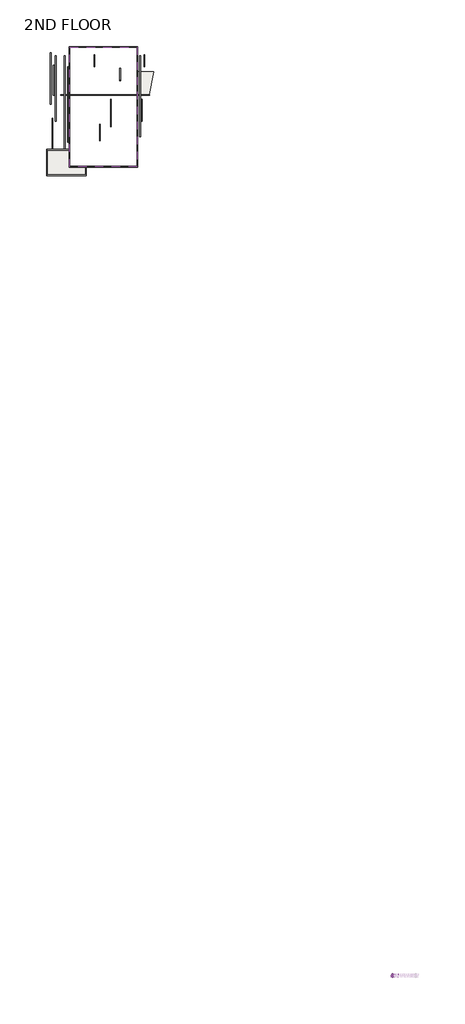
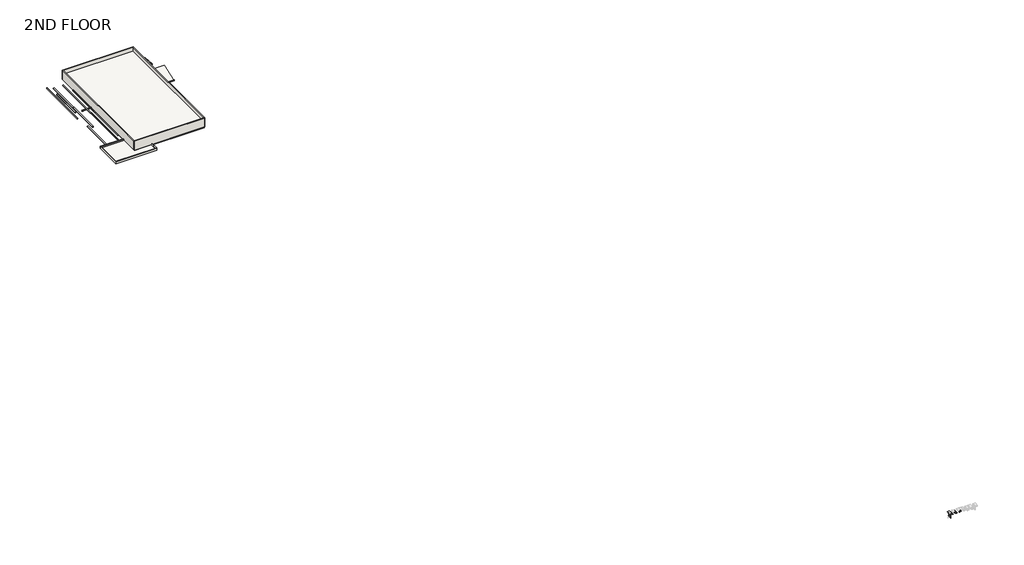
# One storey, part 1 of 2: 20 proxies, 18 beams, 8 walls, 3 slabs.
"""IFC4 building model written with IfcOpenShell, lengths in millimetres."""

import ifcopenshell
import ifcopenshell.guid

model = None  # the IFC model being written
_history = None  # IfcOwnerHistory: only IFC2X3 demands one
_inside = {}  # id of a spatial element -> (the spatial element, [elements in it])
_under = {}  # id of a project, library or spatial element -> (it, [spatial elements below it])
_declared = {}  # id of a project -> (the project, [libraries it declares])
_typed = {}  # id of a type object -> (the type object, [elements of that type])
_made_of = {}  # id of a material, layer set ... -> (it, [elements and type objects made of it])


def new_model(schema):
    """Start an empty IFC model of exactly this schema.

    Asked for "IFC4X3", IfcOpenShell would pick the latest addendum, in which some entities
    have other attributes; the version numbers below select the first issue.
    IFC2X3 requires an IfcOwnerHistory on every rooted entity: one is made here for all.
    """
    global model, _history
    if schema == "IFC4X3":
        model = ifcopenshell.file(schema_version=(4, 3, 0, 0))
    else:
        model = ifcopenshell.file(schema=schema)
    _inside.clear()
    _under.clear()
    _declared.clear()
    _typed.clear()
    _made_of.clear()
    _history = None
    if model.schema == "IFC2X3":
        org = make("IfcOrganization", Name="unknown")
        user = make(
            "IfcPersonAndOrganization",
            ThePerson=make("IfcPerson", FamilyName="unknown"),
            TheOrganization=org,
        )
        app = make(
            "IfcApplication",
            ApplicationDeveloper=org,
            Version="unknown",
            ApplicationFullName="unknown",
            ApplicationIdentifier="unknown",
        )
        _history = make(
            "IfcOwnerHistory",
            OwningUser=user,
            OwningApplication=app,
            ChangeAction="ADDED",
            CreationDate=0,
        )
    return model


def make(cls, **values):
    """One entity of the class cls with the attributes given. An attribute that is None is left unset."""
    return model.create_entity(
        cls, **{name: value for name, value in values.items() if value is not None}
    )


def rooted(cls, **values):
    """An entity with a GlobalId (a new one), such as an element, a storey or a relation."""
    return make(cls, GlobalId=ifcopenshell.guid.new(), OwnerHistory=_history, **values)


def si_unit(unit_type, name, prefix=None):
    """IfcSIUnit, for example si_unit("LENGTHUNIT", "METRE", prefix="MILLI")."""
    return make("IfcSIUnit", UnitType=unit_type, Prefix=prefix, Name=name)


def assignment(units):
    """IfcUnitAssignment: the units of a project."""
    return None if units is None else make("IfcUnitAssignment", Units=units)


def point(xyz):
    """IfcCartesianPoint."""
    return None if xyz is None else make("IfcCartesianPoint", Coordinates=xyz)


def direction(xyz):
    """IfcDirection."""
    return None if xyz is None else make("IfcDirection", DirectionRatios=xyz)


def frame(location, z_axis=None, x_axis=None):
    """IfcAxis2Placement3D, a coordinate frame: its origin and axes. An axis left out is left unset."""
    return make(
        "IfcAxis2Placement3D",
        Location=point(location),
        Axis=direction(z_axis),
        RefDirection=direction(x_axis),
    )


def frame_2d(location, x_axis=None):
    """IfcAxis2Placement2D, a coordinate frame in the plane: its origin and x axis."""
    return make(
        "IfcAxis2Placement2D", Location=point(location), RefDirection=direction(x_axis)
    )


def origin():
    """The frame at (0, 0, 0) with its axes left unset."""
    return frame((0.0, 0.0, 0.0))


def place(relative_to, where):
    """IfcLocalPlacement: puts the frame where relative to a parent placement (None: the world)."""
    return make(
        "IfcLocalPlacement", PlacementRelTo=relative_to, RelativePlacement=where
    )


def context(
    kind, dimensions, precision=None, world=None, true_north=None, identifier=None
):
    """IfcGeometricRepresentationContext, for example the 3D "Model" context."""
    return make(
        "IfcGeometricRepresentationContext",
        ContextIdentifier=identifier,
        ContextType=kind,
        CoordinateSpaceDimension=dimensions,
        Precision=precision,
        WorldCoordinateSystem=world,
        TrueNorth=true_north,
    )


def project(units=None, contexts=None):
    """IfcProject with its units and contexts."""
    return rooted(
        "IfcProject",
        Name="project",
        RepresentationContexts=contexts,
        UnitsInContext=assignment(units),
    )


def spatial(cls, under=None, at=None, **own):
    """A site, building, storey or space (cls), placed at a placement, below another one or the project."""
    s = rooted(cls, ObjectPlacement=at, **own)
    if under is not None:
        _under.setdefault(under.id(), (under, []))[1].append(s)
    return s


def polyline(points):
    """IfcPolyline through the points."""
    return make("IfcPolyline", Points=[point(p) for p in points])


def circle_curve(where, radius):
    """IfcCircle in the frame where."""
    return make("IfcCircle", Position=where, Radius=radius)


def trimmed(basis, trim1, trim2, sense, master):
    """IfcTrimmedCurve: the piece of a basis curve between two trims."""
    return make(
        "IfcTrimmedCurve",
        BasisCurve=basis,
        Trim1=trim1,
        Trim2=trim2,
        SenseAgreement=sense,
        MasterRepresentation=master,
    )


def segment(curve, same_sense, transition):
    """IfcCompositeCurveSegment."""
    return make(
        "IfcCompositeCurveSegment",
        Transition=transition,
        SameSense=same_sense,
        ParentCurve=curve,
    )


def composite_curve(segments, self_intersect=None):
    """IfcCompositeCurve: segments joined end to end."""
    return make("IfcCompositeCurve", Segments=segments, SelfIntersect=self_intersect)


def outline(outer, holes=None, kind="AREA"):
    """IfcArbitraryClosedProfileDef: a profile drawn as a closed curve; with holes, ...WithVoids."""
    if holes is None:
        return make("IfcArbitraryClosedProfileDef", ProfileType=kind, OuterCurve=outer)
    return make(
        "IfcArbitraryProfileDefWithVoids",
        ProfileType=kind,
        OuterCurve=outer,
        InnerCurves=holes,
    )


def extrude(swept, where, along, depth):
    """IfcExtrudedAreaSolid: the profile swept, set in the frame where, extruded along a direction by depth."""
    return make(
        "IfcExtrudedAreaSolid",
        SweptArea=swept,
        Position=where,
        ExtrudedDirection=direction(along),
        Depth=depth,
    )


def faces_of(points, faces, orient=None, outer=None):
    """IfcFace entities. A face is a list of loops; a loop is a list of indices into points, from 0.

    orient and outer hold one flag for each loop. By default every Orientation is true, the
    first loop of a face is its IfcFaceOuterBound and the others are IfcFaceBound.
    """
    made = []
    for i, loops in enumerate(faces):
        bounds = []
        for j, loop in enumerate(loops):
            is_outer = j == 0 if outer is None else outer[i][j]
            bounds.append(
                make(
                    "IfcFaceOuterBound" if is_outer else "IfcFaceBound",
                    Bound=make("IfcPolyLoop", Polygon=[points[k] for k in loop]),
                    Orientation=True if orient is None else orient[i][j],
                )
            )
        made.append(make("IfcFace", Bounds=bounds))
    return made


def faceted_brep(points, faces, orient=None, outer=None, voids=None):
    """IfcFacetedBrep: a solid bounded by flat faces; with voids (closed shells), ...WithVoids."""
    shared = [point(p) for p in points]
    hull = make("IfcClosedShell", CfsFaces=faces_of(shared, faces, orient, outer))
    if voids is None:
        return make("IfcFacetedBrep", Outer=hull)
    return make(
        "IfcFacetedBrepWithVoids",
        Outer=hull,
        Voids=[
            make(cls, CfsFaces=faces_of(shared, fs, o, b)) for cls, fs, o, b in voids
        ],
    )


def shape(context_of_items, identifier, shape_type, items):
    """IfcShapeRepresentation: the items that make up one representation, for example the "Body"."""
    return make(
        "IfcShapeRepresentation",
        ContextOfItems=context_of_items,
        RepresentationIdentifier=identifier,
        RepresentationType=shape_type,
        Items=items,
    )


def source(mapping_origin, context_of_items, identifier, shape_type, items):
    """IfcRepresentationMap: a shape defined once, which mapped items show again and again."""
    return make(
        "IfcRepresentationMap",
        MappingOrigin=mapping_origin,
        MappedRepresentation=shape(context_of_items, identifier, shape_type, items),
    )


def transform(
    local_origin,
    x_axis=None,
    y_axis=None,
    z_axis=None,
    scale=None,
    scale2=None,
    scale3=None,
    uniform=True,
):
    """IfcCartesianTransformationOperator3D, or its non-uniform kind. x_axis, y_axis, z_axis: its Axis1, 2, 3."""
    if uniform:
        return make(
            "IfcCartesianTransformationOperator3D",
            Axis1=direction(x_axis),
            Axis2=direction(y_axis),
            LocalOrigin=point(local_origin),
            Scale=scale,
            Axis3=direction(z_axis),
        )
    return make(
        "IfcCartesianTransformationOperator3DnonUniform",
        Axis1=direction(x_axis),
        Axis2=direction(y_axis),
        LocalOrigin=point(local_origin),
        Scale=scale,
        Axis3=direction(z_axis),
        Scale2=scale2,
        Scale3=scale3,
    )


def mapped(mapping_source, mapping_target):
    """IfcMappedItem: shows the shape of a source again, moved by a transform."""
    return make(
        "IfcMappedItem", MappingSource=mapping_source, MappingTarget=mapping_target
    )


def made_of(thing, what):
    """Note that an element or type object is made of a material, layer set ...; save() writes the relation."""
    if what is not None:
        _made_of.setdefault(what.id(), (what, []))[1].append(thing)
    return thing


def element(
    cls,
    number,
    at=None,
    inside=None,
    cuts=None,
    type_object=None,
    material=None,
    context=None,
    identifier="Body",
    shape_type=None,
    held_by="IfcProductDefinitionShape",
    body=None,
    shapes=None,
    **own,
):
    """One element of the class cls, such as IfcWall. Its Tag is "e" and its number.

    at: its placement. inside: the storey or other place that contains it. cuts: it is an
    opening in that element (IfcRelVoidsElement). A single representation is given by context,
    identifier, shape_type and body (its items); several are given by shapes. held_by: the class
    of the entity that holds the representations. save() writes the other relations.
    """
    e = rooted(cls, Tag="e%d" % number, ObjectPlacement=at, **own)
    if body is not None:
        shapes = [shape(context, identifier, shape_type, body)]
    if shapes is not None:
        e.Representation = make(held_by, Representations=shapes)
    if inside is not None:
        _inside.setdefault(inside.id(), (inside, []))[1].append(e)
    if cuts is not None:
        rooted(
            "IfcRelVoidsElement", RelatingBuildingElement=cuts, RelatedOpeningElement=e
        )
    if type_object is not None:
        _typed.setdefault(type_object.id(), (type_object, []))[1].append(e)
    return made_of(e, material)


def aggregate(whole, parts):
    """IfcRelAggregates: a whole, such as a stair, and the parts it consists of."""
    return rooted("IfcRelAggregates", RelatingObject=whole, RelatedObjects=parts)


def save(model, path):
    """Write the relations noted so far, then the file.

    IfcRelAggregates (storeys below a building ...), IfcRelContainedInSpatialStructure (elements
    in a storey), IfcRelDefinesByType, IfcRelAssociatesMaterial and IfcRelDeclares: one each for
    every whole, place, type object, material and project.
    """
    for whole, parts in _under.values():
        aggregate(whole, parts)
    for where, things in _inside.values():
        rooted(
            "IfcRelContainedInSpatialStructure",
            RelatedElements=things,
            RelatingStructure=where,
        )
    for kind, things in _typed.values():
        rooted("IfcRelDefinesByType", RelatedObjects=things, RelatingType=kind)
    for what, things in _made_of.values():
        rooted("IfcRelAssociatesMaterial", RelatedObjects=things, RelatingMaterial=what)
    for by, libraries in _declared.values():
        rooted("IfcRelDeclares", RelatingContext=by, RelatedDefinitions=libraries)
    model.write(path)


def dimension_lumber_10x10_beam_780dcf97(model_context):
    return source(origin(), model_context, "Body", "SweptSolid", [
        extrude(outline(polyline([(3429.0, 117.475), (3429.0, -117.475), (-3429.0, -117.475), (-3429.0, 117.475), (3429.0, 117.475)])), frame((0.0, 0.0, -117.475), z_axis=(0.0, 0.0, 1.0), x_axis=(1.0, 0.0, 0.0)), (0.0, 0.0, 1.0), 234.95),
    ])


def dimension_lumber_10x10_beam_a659b46f(model_context):
    return source(origin(), model_context, "Body", "SweptSolid", [
        extrude(outline(polyline([(11658.6, 117.475), (11658.6, -117.475), (-11658.6, -117.475), (-11658.6, 117.475), (11658.6, 117.475)])), frame((0.0, 0.0, -117.475), z_axis=(0.0, 0.0, 1.0), x_axis=(1.0, 0.0, 0.0)), (0.0, 0.0, 1.0), 234.95),
    ])


def dimension_lumber_10x10_beam_82f4ea42(model_context):
    return source(origin(), model_context, "Body", "SweptSolid", [
        extrude(outline(polyline([(4648.2, 117.475), (4648.2, -117.475), (-4648.2, -117.475), (-4648.2, 117.475), (4648.2, 117.475)])), frame((0.0, 0.0, -117.475), z_axis=(0.0, 0.0, 1.0), x_axis=(1.0, 0.0, 0.0)), (0.0, 0.0, 1.0), 234.95),
    ])


def dimension_lumber_10x10_beam_babce44f(model_context):
    return source(origin(), model_context, "Body", "SweptSolid", [
        extrude(outline(polyline([(7924.8, 117.475), (7924.8, -117.475), (-7924.8, -117.475), (-7924.8, 117.475), (7924.8, 117.475)])), frame((0.0, 0.0, -117.475), z_axis=(0.0, 0.0, 1.0), x_axis=(1.0, 0.0, 0.0)), (0.0, 0.0, 1.0), 234.95),
    ])


def dimension_lumber_10x10_beam_47096931(model_context):
    return source(origin(), model_context, "Body", "SweptSolid", [
        extrude(outline(polyline([(10420.9864513, 117.475), (10420.9864513, -117.475), (-10420.9864513, -117.475), (-10420.9864513, 117.475), (10420.9864513, 117.475)])), frame((0.0, 0.0, -117.475), z_axis=(0.0, 0.0, 1.0), x_axis=(1.0, 0.0, 0.0)), (0.0, 0.0, 1.0), 234.95),
    ])


def dimension_lumber_10x10_beam_db3298f4(model_context):
    return source(origin(), model_context, "Body", "SweptSolid", [
        extrude(outline(polyline([(12496.8, 117.475), (12496.8, -117.475), (-12496.8, -117.475), (-12496.8, 117.475), (12496.8, 117.475)])), frame((0.0, 0.0, -117.475), z_axis=(0.0, 0.0, 1.0), x_axis=(1.0, 0.0, 0.0)), (0.0, 0.0, 1.0), 234.95),
    ])


def dimension_lumber_10x10_beam_470fd3cf(model_context):
    return source(origin(), model_context, "Body", "SweptSolid", [
        extrude(outline(polyline([(1876.3363558, 117.475), (1876.3363558, -117.475), (-1876.3363558, -117.475), (-1876.3363558, 117.475), (1876.3363558, 117.475)])), frame((0.0, 0.0, -117.475), z_axis=(0.0, 0.0, 1.0), x_axis=(1.0, 0.0, 0.0)), (0.0, 0.0, 1.0), 234.95),
    ])


def dimension_lumber_10x10_beam_1dfca716(model_context):
    return source(origin(), model_context, "Body", "SweptSolid", [
        extrude(outline(polyline([(10094.9494295, 117.475), (10094.9494295, -117.475), (-10094.9494295, -117.475), (-10094.9494295, 117.475), (10094.9494295, 117.475)])), frame((0.0, 0.0, -117.475), z_axis=(0.0, 0.0, 1.0), x_axis=(1.0, 0.0, 0.0)), (0.0, 0.0, 1.0), 234.95),
    ])


def dimension_lumber_10x10_beam_bd205abd(model_context):
    return source(origin(), model_context, "Body", "SweptSolid", [
        extrude(outline(polyline([(14564.075555, 117.475), (14564.075555, -117.475), (-14467.238055, -117.475), (-14467.238055, 117.475), (14564.075555, 117.475)])), frame((0.0, 0.0, -117.475), z_axis=(0.0, 0.0, 1.0), x_axis=(1.0, 0.0, 0.0)), (0.0, 0.0, 1.0), 234.95),
    ])


def dimension_lumber_10x10_beam_e017d86a(model_context):
    return source(origin(), model_context, "Body", "SweptSolid", [
        extrude(outline(polyline([(4267.2, 117.475), (4267.2, -117.475), (-4267.2, -117.475), (-4267.2, 117.475), (4267.2, 117.475)])), frame((0.0, 0.0, -117.475), z_axis=(0.0, 0.0, 1.0), x_axis=(1.0, 0.0, 0.0)), (0.0, 0.0, 1.0), 234.95),
    ])


def dimension_lumber_10x10_beam_f930df24(model_context):
    return source(origin(), model_context, "Body", "SweptSolid", [
        extrude(outline(polyline([(2514.6, 117.475), (2514.6, -117.475), (-2514.6, -117.475), (-2514.6, 117.475), (2514.6, 117.475)])), frame((0.0, 0.0, -117.475), z_axis=(0.0, 0.0, 1.0), x_axis=(1.0, 0.0, 0.0)), (0.0, 0.0, 1.0), 234.95),
    ])


def w_wide_flange_w12x26_f67572b3(model_context):
    return source(origin(), model_context, "Body", "SweptSolid", [
        extrude(outline(composite_curve([segment(polyline([(82.4011719, -145.5539063), (82.4011719, -155.178125), (-82.4011719, -155.178125), (-82.4011719, -145.5539063), (-20.2902344, -145.5539063)]), True, "CONTINUOUS"), segment(trimmed(circle_curve(frame_2d((-20.2902344, -128.190625)), 17.3632812), [point((-20.2902344, -145.5539063))], [point((-2.9269531, -128.190625))], True, "CARTESIAN"), True, "CONTINUOUS"), segment(polyline([(-2.9269531, -128.190625), (-2.9269531, 128.190625)]), True, "CONTINUOUS"), segment(trimmed(circle_curve(frame_2d((-20.2902344, 128.190625)), 17.3632812), [point((-2.9269531, 128.190625))], [point((-20.2902344, 145.5539062))], True, "CARTESIAN"), True, "CONTINUOUS"), segment(polyline([(-20.2902344, 145.5539062), (-82.4011719, 145.5539062), (-82.4011719, 155.178125), (82.4011719, 155.178125), (82.4011719, 145.5539062), (20.2902344, 145.5539062)]), True, "CONTINUOUS"), segment(trimmed(circle_curve(frame_2d((20.2902344, 128.190625)), 17.3632812), [point((20.2902344, 145.5539062))], [point((2.9269531, 128.190625))], True, "CARTESIAN"), True, "CONTINUOUS"), segment(polyline([(2.9269531, 128.190625), (2.9269531, -128.190625)]), True, "CONTINUOUS"), segment(trimmed(circle_curve(frame_2d((20.2902344, -128.190625)), 17.3632812), [point((2.9269531, -128.190625))], [point((20.2902344, -145.5539063))], True, "CARTESIAN"), True, "CONTINUOUS"), segment(polyline([(20.2902344, -145.5539063), (82.4011719, -145.5539063)]), True, "CONTINUOUS")], self_intersect=False)), frame((-18489.1180586, 0.0, 0.0), z_axis=(1.0, 0.0, 0.0), x_axis=(0.0, 1.0, 0.0)), (0.0, 0.0, 1.0), 36978.2361173),
    ])


def w_wide_flange_w12x26_0a813f0e(model_context):
    return source(origin(), model_context, "Body", "SweptSolid", [
        extrude(outline(composite_curve([segment(polyline([(82.4011719, -145.5539063), (82.4011719, -155.178125), (-82.4011719, -155.178125), (-82.4011719, -145.5539063), (-20.2902344, -145.5539063)]), True, "CONTINUOUS"), segment(trimmed(circle_curve(frame_2d((-20.2902344, -128.190625)), 17.3632812), [point((-20.2902344, -145.5539063))], [point((-2.9269531, -128.190625))], True, "CARTESIAN"), True, "CONTINUOUS"), segment(polyline([(-2.9269531, -128.190625), (-2.9269531, 128.190625)]), True, "CONTINUOUS"), segment(trimmed(circle_curve(frame_2d((-20.2902344, 128.190625)), 17.3632812), [point((-2.9269531, 128.190625))], [point((-20.2902344, 145.5539062))], True, "CARTESIAN"), True, "CONTINUOUS"), segment(polyline([(-20.2902344, 145.5539062), (-82.4011719, 145.5539062), (-82.4011719, 155.178125), (82.4011719, 155.178125), (82.4011719, 145.5539062), (20.2902344, 145.5539062)]), True, "CONTINUOUS"), segment(trimmed(circle_curve(frame_2d((20.2902344, 128.190625)), 17.3632812), [point((20.2902344, 145.5539062))], [point((2.9269531, 128.190625))], True, "CARTESIAN"), True, "CONTINUOUS"), segment(polyline([(2.9269531, 128.190625), (2.9269531, -128.190625)]), True, "CONTINUOUS"), segment(trimmed(circle_curve(frame_2d((20.2902344, -128.190625)), 17.3632812), [point((2.9269531, -128.190625))], [point((20.2902344, -145.5539063))], True, "CARTESIAN"), True, "CONTINUOUS"), segment(polyline([(20.2902344, -145.5539063), (82.4011719, -145.5539063)]), True, "CONTINUOUS")], self_intersect=False)), frame((-25624.0113662, 0.0, 0.0), z_axis=(1.0, 0.0, 0.0), x_axis=(0.0, 1.0, 0.0)), (0.0, 0.0, 1.0), 27573.8603238),
    ])


def w_wide_flange_w12x26_89544ef1(model_context):
    return source(origin(), model_context, "Body", "SweptSolid", [
        extrude(outline(composite_curve([segment(polyline([(82.4011719, -145.5539063), (82.4011719, -155.178125), (-82.4011719, -155.178125), (-82.4011719, -145.5539063), (-20.2902344, -145.5539063)]), True, "CONTINUOUS"), segment(trimmed(circle_curve(frame_2d((-20.2902344, -128.190625)), 17.3632812), [point((-20.2902344, -145.5539063))], [point((-2.9269531, -128.190625))], True, "CARTESIAN"), True, "CONTINUOUS"), segment(polyline([(-2.9269531, -128.190625), (-2.9269531, 128.190625)]), True, "CONTINUOUS"), segment(trimmed(circle_curve(frame_2d((-20.2902344, 128.190625)), 17.3632812), [point((-2.9269531, 128.190625))], [point((-20.2902344, 145.5539062))], True, "CARTESIAN"), True, "CONTINUOUS"), segment(polyline([(-20.2902344, 145.5539062), (-82.4011719, 145.5539062), (-82.4011719, 155.178125), (82.4011719, 155.178125), (82.4011719, 145.5539062), (20.2902344, 145.5539062)]), True, "CONTINUOUS"), segment(trimmed(circle_curve(frame_2d((20.2902344, 128.190625)), 17.3632812), [point((20.2902344, 145.5539062))], [point((2.9269531, 128.190625))], True, "CARTESIAN"), True, "CONTINUOUS"), segment(polyline([(2.9269531, 128.190625), (2.9269531, -128.190625)]), True, "CONTINUOUS"), segment(trimmed(circle_curve(frame_2d((20.2902344, -128.190625)), 17.3632812), [point((2.9269531, -128.190625))], [point((20.2902344, -145.5539063))], True, "CARTESIAN"), True, "CONTINUOUS"), segment(polyline([(20.2902344, -145.5539063), (82.4011719, -145.5539063)]), True, "CONTINUOUS")], self_intersect=False)), frame((-18440.6993086, 0.0, 0.0), z_axis=(1.0, 0.0, 0.0), x_axis=(0.0, 1.0, 0.0)), (0.0, 0.0, 1.0), 36978.2361173),
    ])


def generic_models_1_generic_models_1_05f3df34(model_context):
    return source(origin(), model_context, "Body", "SweptSolid", [
        extrude(outline(polyline([(49784.0, 0.0), (49695.1, 0.0), (49695.1, 1219.2), (49784.0, 1219.2), (49784.0, 0.0)])), frame((0.0, 0.0, 3048.0), z_axis=(0.0, 0.0, 1.0), x_axis=(1.0, 0.0, 0.0)), (0.0, 0.0, 1.0), 38.1),
    ])


def generic_models_157_generic_models_1_b3b9a6c0(model_context):
    return source(origin(), model_context, "Body", "SweptSolid", [
        extrude(outline(polyline([(47363.0625, 1219.2), (47363.0625, 0.0), (47347.1875, 0.0), (47347.1875, 1219.2), (47363.0625, 1219.2)])), frame((0.0, 0.0, 4267.2), z_axis=(0.0, 0.0, 1.0), x_axis=(1.0, 0.0, 0.0)), (0.0, 0.0, 1.0), 1123.95),
    ])


def generic_models_14_generic_models_1_e8c90d4c(model_context):
    return source(origin(), model_context, "Body", "SweptSolid", [
        extrude(outline(polyline([(2277.1204978, 49799.875), (2239.0204978, 49799.875), (2239.0204978, 49825.275), (2240.6079978, 49825.275), (2240.6079978, 49801.4625), (2277.1204978, 49801.4625), (2277.1204978, 49799.875)])), frame((0.0, 0.0, 0.0), z_axis=(0.0, 1.0, 0.0), x_axis=(0.0, 0.0, 1.0)), (0.0, 0.0, 1.0), 1219.2),
    ])


def generic_models_22_generic_models_1_e5767157(model_context):
    return source(origin(), model_context, "Body", "SweptSolid", [
        extrude(outline(polyline([(2409.6091, 49800.66875), (2409.6091, 49799.875), (2407.0592364, 49799.875), (2405.4618473, 49749.075), (2404.6631527, 49749.075), (2403.0657636, 49799.875), (2400.5159, 49799.875), (2400.5159, 49800.66875), (2409.6091, 49800.66875)])), frame((0.0, 565.15, 0.0), z_axis=(0.0, 1.0, 0.0), x_axis=(0.0, 0.0, 1.0)), (0.0, 0.0, 1.0), 12.7),
    ])


def generic_models_226_generic_models_1_7dc37832(model_context):
    return source(origin(), model_context, "Body", "SweptSolid", [
        extrude(outline(polyline([(5263.35625, 49733.4159), (5263.35625, 49742.5091), (5264.15, 49742.5091), (5264.15, 49739.9592364), (5314.95, 49738.3618473), (5314.95, 49737.5631527), (5264.15, 49735.9657636), (5264.15, 49733.4159), (5263.35625, 49733.4159)])), frame((0.0, 565.15, 0.0), z_axis=(0.0, 1.0, 0.0), x_axis=(0.0, 0.0, 1.0)), (0.0, 0.0, 1.0), 12.7),
    ])


def generic_models_202_generic_models_1_0ad20a8b(model_context):
    return source(origin(), model_context, "Body", "SweptSolid", [
        extrude(outline(polyline([(2253.330428, 49813.3451407), (2242.217928, 49813.3451407), (2242.217928, 49826.0451407), (2234.280428, 49828.9341545), (2234.280428, 50422.9451407), (2253.330428, 50422.9451407), (2253.330428, 49813.3451407)])), frame((0.0, 0.0, 0.0), z_axis=(0.0, 1.0, 0.0), x_axis=(0.0, 0.0, 1.0)), (0.0, 0.0, 1.0), 1219.2),
    ])


def generic_models_239_generic_models_46_95e6735a(model_context):
    return source(origin(), model_context, "Body", "SweptSolid", [
        extrude(outline(polyline([(50347.5625, 0.0), (49691.4320511, 0.0), (49691.4320511, 1219.2), (50347.5625, 1219.2), (50347.5625, 0.0)])), frame((0.0, 0.0, 5505.7509163), z_axis=(0.0, 0.0, 1.0), x_axis=(1.0, 0.0, 0.0)), (0.0, 0.0, 1.0), 1.5875),
    ])


def generic_models_233_generic_models_1_ae5bae41(model_context):
    return source(origin(), model_context, "Body", "SweptSolid", [
        extrude(outline(polyline([(48564.8, 0.0), (48475.9, 0.0), (48475.9, 1219.2), (48564.8, 1219.2), (48564.8, 0.0)])), frame((0.0, 0.0, 5467.35), z_axis=(0.0, 0.0, 1.0), x_axis=(1.0, 0.0, 0.0)), (0.0, 0.0, 1.0), 38.1),
    ])


def generic_models_237_generic_models_65_1df05f16(model_context):
    return source(origin(), model_context, "Body", "SweptSolid", [
        extrude(outline(polyline([(48469.55, 592.1375), (48469.55, 630.2375), (49128.3625, 630.2375), (49128.3625, 592.1375), (48469.55, 592.1375)])), frame((0.0, 0.0, 5507.83125), z_axis=(0.0, 0.0, 1.0), x_axis=(1.0, 0.0, 0.0)), (0.0, 0.0, 1.0), 139.7),
    ])


def generic_models_240_generic_models_1_611786cf(model_context):
    return source(origin(), model_context, "Body", "SweptSolid", [
        extrude(outline(polyline([(49128.3625, 1219.2), (49128.3625, 0.0), (48469.55, 0.0), (48469.55, 1219.2), (49128.3625, 1219.2)])), frame((0.0, 0.0, 5649.9125), z_axis=(0.0, 0.0, 1.0), x_axis=(1.0, 0.0, 0.0)), (0.0, 0.0, 1.0), 19.05),
    ])


model = new_model("IFC4")

# Units and contexts
model_context = context("Model", 3, world=origin())
ifc_project = project(units=[si_unit("LENGTHUNIT", "METRE", prefix="MILLI")], contexts=[model_context])

# Site, building, storey
site = spatial("IfcSite", under=ifc_project)
building = spatial("IfcBuilding", under=site)
storey = spatial("IfcBuildingStorey", under=building, Name="2ND FLOOR", Elevation=3657.6)

# Beams
placement = place(None, origin())
dimension_lumber_10x10_beam_shape = dimension_lumber_10x10_beam_780dcf97(model_context)
element("IfcBeam", 1, ObjectType="Dimension Lumber : 10x10 - BEAM", at=placement, inside=storey, context=model_context, shape_type="MappedRepresentation", body=[
    mapped(dimension_lumber_10x10_beam_shape, transform((-31351.8083583, 267736.5959777, 4098.925), x_axis=(0.0, 1.0, 0.0), y_axis=(-1.0, 0.0, 0.0), z_axis=(0.0, 0.0, 1.0))),
])
dimension_lumber_10x10_beam_2_shape = dimension_lumber_10x10_beam_a659b46f(model_context)
element("IfcBeam", 2, ObjectType="Dimension Lumber : 10x10 - BEAM", at=placement, inside=storey, context=model_context, shape_type="MappedRepresentation", body=[
    mapped(dimension_lumber_10x10_beam_2_shape, transform((-54174.023811, 269565.3959777, 4098.925), x_axis=(0.0, 1.0, 0.0), y_axis=(-1.0, 0.0, 0.0), z_axis=(0.0, 0.0, 1.0))),
])
dimension_lumber_10x10_beam_3_shape = dimension_lumber_10x10_beam_82f4ea42(model_context)
element("IfcBeam", 3, ObjectType="Dimension Lumber : 10x10 - BEAM", at=placement, inside=storey, context=model_context, shape_type="MappedRepresentation", body=[
    mapped(dimension_lumber_10x10_beam_3_shape, transform((-58593.623811, 277032.9959777, 4098.925), x_axis=(0.0, 1.0, 0.0), y_axis=(-1.0, 0.0, 0.0), z_axis=(0.0, 0.0, 1.0))),
])
element("IfcBeam", 4, ObjectType="Dimension Lumber : 10x10 - BEAM", at=placement, inside=storey, context=model_context, shape_type="MappedRepresentation", body=[
    mapped(dimension_lumber_10x10_beam_3_shape, transform((-58989.4061381, 260573.7959777, 4098.925), x_axis=(0.0, 1.0, 0.0), y_axis=(-1.0, 0.0, 0.0), z_axis=(0.0, 0.0, 1.0))),
])
dimension_lumber_10x10_beam_4_shape = dimension_lumber_10x10_beam_babce44f(model_context)
element("IfcBeam", 5, ObjectType="Dimension Lumber : 10x10 - BEAM", at=placement, inside=storey, context=model_context, shape_type="MappedRepresentation", body=[
    mapped(dimension_lumber_10x10_beam_4_shape, transform((-59508.023811, 277566.3959777, 4098.925), x_axis=(0.0, 1.0, 0.0), y_axis=(-1.0, 0.0, 0.0), z_axis=(0.0, 0.0, 1.0))),
])
dimension_lumber_10x10_beam_5_shape = dimension_lumber_10x10_beam_47096931(model_context)
element("IfcBeam", 6, ObjectType="Dimension Lumber : 10x10 - BEAM", at=placement, inside=storey, context=model_context, shape_type="MappedRepresentation", body=[
    mapped(dimension_lumber_10x10_beam_5_shape, transform((-43244.9562094, 250288.6950863, 3844.925), x_axis=(1.0, 0.0, 0.0), y_axis=(0.0, 1.0, 0.0), z_axis=(0.0, 0.0, 1.0))),
])
element("IfcBeam", 7, ObjectType="Dimension Lumber : 10x10 - BEAM", at=placement, inside=storey, context=model_context, shape_type="MappedRepresentation", body=[
    mapped(dimension_lumber_10x10_beam_5_shape, transform((-43244.9562094, 287271.6937036, 3844.925), x_axis=(1.0, 0.0, 0.0), y_axis=(0.0, 1.0, 0.0), z_axis=(0.0, 0.0, 1.0))),
])
dimension_lumber_10x10_beam_6_shape = dimension_lumber_10x10_beam_db3298f4(model_context)
element("IfcBeam", 8, ObjectType="Dimension Lumber : 10x10 - BEAM", at=placement, inside=storey, context=model_context, shape_type="MappedRepresentation", body=[
    mapped(dimension_lumber_10x10_beam_6_shape, transform((-31923.623811, 272079.9959777, 4098.925), x_axis=(0.0, 1.0, 0.0), y_axis=(-1.0, 0.0, 0.0), z_axis=(0.0, 0.0, 1.0))),
])
dimension_lumber_10x10_beam_7_shape = dimension_lumber_10x10_beam_470fd3cf(model_context)
element("IfcBeam", 9, ObjectType="Dimension Lumber : 10x10 - BEAM", at=placement, inside=storey, context=model_context, shape_type="MappedRepresentation", body=[
    mapped(dimension_lumber_10x10_beam_7_shape, transform((-30552.023811, 283024.5607339, 3972.1944014), x_axis=(0.0, 0.9977067345863507, -0.06768509260569218), y_axis=(-1.0, 0.0, 0.0), z_axis=(0.0, 0.06768509260569247, 0.9977067345863507))),
])
element("IfcBeam", 10, ObjectType="Dimension Lumber : 10x10 - BEAM", at=placement, inside=storey, context=model_context, shape_type="MappedRepresentation", body=[
    mapped(dimension_lumber_10x10_beam_7_shape, transform((-46009.1160671, 283024.5607339, 3972.1944014), x_axis=(0.0, 0.9977067345863507, -0.06768509260569218), y_axis=(-1.0, 0.0, 0.0), z_axis=(0.0, 0.06768509260569247, 0.9977067345863507))),
])
element("IfcBeam", 11, ObjectType="Dimension Lumber : 10x10 - BEAM", at=placement, inside=storey, context=model_context, shape_type="MappedRepresentation", body=[
    mapped(dimension_lumber_10x10_beam_7_shape, transform((-38058.8151936, 278801.0732117, 3972.1944014), x_axis=(0.0, 0.9977067345863507, -0.06768509260569218), y_axis=(-1.0, 0.0, 0.0), z_axis=(0.0, 0.06768509260569247, 0.9977067345863507))),
])
dimension_lumber_10x10_beam_8_shape = dimension_lumber_10x10_beam_1dfca716(model_context)
element("IfcBeam", 12, ObjectType="Dimension Lumber : 10x10 - BEAM", at=placement, inside=storey, context=model_context, shape_type="MappedRepresentation", body=[
    mapped(dimension_lumber_10x10_beam_8_shape, transform((-57984.023811, 274481.8465482, 4098.925), x_axis=(0.0, 1.0, 0.0), y_axis=(-1.0, 0.0, 0.0), z_axis=(0.0, 0.0, 1.0))),
])
dimension_lumber_10x10_beam_9_shape = dimension_lumber_10x10_beam_bd205abd(model_context)
element("IfcBeam", 13, ObjectType="Dimension Lumber : 10x10 - BEAM", at=placement, inside=storey, context=model_context, shape_type="MappedRepresentation", body=[
    mapped(dimension_lumber_10x10_beam_9_shape, transform((-55240.823811, 270012.7204227, 4098.925), x_axis=(0.0, 1.0, 0.0), y_axis=(-1.0, 0.0, 0.0), z_axis=(0.0, 0.0, 1.0))),
])
dimension_lumber_10x10_beam_10_shape = dimension_lumber_10x10_beam_e017d86a(model_context)
element("IfcBeam", 14, ObjectType="Dimension Lumber : 10x10 - BEAM", at=placement, inside=storey, context=model_context, shape_type="MappedRepresentation", body=[
    mapped(dimension_lumber_10x10_beam_10_shape, transform((-40934.9769456, 266898.3959777, 4098.925), x_axis=(0.0, 1.0, 0.0), y_axis=(-1.0, 0.0, 0.0), z_axis=(0.0, 0.0, 1.0))),
])
dimension_lumber_10x10_beam_11_shape = dimension_lumber_10x10_beam_f930df24(model_context)
element("IfcBeam", 15, ObjectType="Dimension Lumber : 10x10 - BEAM", at=placement, inside=storey, context=model_context, shape_type="MappedRepresentation", body=[
    mapped(dimension_lumber_10x10_beam_11_shape, transform((-44340.4912327, 260860.7569797, 3972.0749209), x_axis=(0.0, 0.9987238056006686, -0.05050505050505233), y_axis=(-1.0, 0.0, 0.0), z_axis=(0.0, 0.05050505050505244, 0.9987238056006686))),
])
w_wide_flange_w12x26_shape = w_wide_flange_w12x26_f67572b3(model_context)
element("IfcBeam", 16, ObjectType="W-Wide Flange : W12X26", at=placement, inside=storey, context=model_context, shape_type="MappedRepresentation", body=[
    mapped(w_wide_flange_w12x26_shape, transform((-53686.5801606, 268727.0131449, 3807.221875), x_axis=(0.0, -1.0, 0.0), y_axis=(1.0, 0.0, 0.0), z_axis=(0.0, 0.0, 1.0))),
])
w_wide_flange_w12x26_2_shape = w_wide_flange_w12x26_0a813f0e(model_context)
element("IfcBeam", 17, ObjectType="W-Wide Flange : W12X26", at=placement, inside=storey, context=model_context, shape_type="MappedRepresentation", body=[
    mapped(w_wide_flange_w12x26_2_shape, transform((-30876.3646415, 272462.0550317, 3807.221875), x_axis=(1.0, 0.0, 0.0), y_axis=(0.0, 1.0, 0.0), z_axis=(0.0, 0.0, 1.0))),
])
w_wide_flange_w12x26_3_shape = w_wide_flange_w12x26_89544ef1(model_context)
element("IfcBeam", 18, ObjectType="W-Wide Flange : W12X26", at=placement, inside=storey, context=model_context, shape_type="MappedRepresentation", body=[
    mapped(w_wide_flange_w12x26_3_shape, transform((-32792.2943075, 268775.4318949, 3807.2455094), x_axis=(0.0, 1.0, 0.0), y_axis=(-0.9998476951563913, 0.0, -0.017452406437283494), z_axis=(-0.017452406437283494, 0.0, 0.9998476951563913))),
])

# Proxies
generic_models_1_generic_models_1_shape = generic_models_1_generic_models_1_05f3df34(model_context)
element("IfcBuildingElementProxy", 19, Name="Generic Models 155 : Generic Models 1", ObjectType="Generic Models 155 : Generic Models 1", at=placement, inside=storey, context=model_context, shape_type="MappedRepresentation", body=[
    mapped(generic_models_1_generic_models_1_shape, transform((-3657.6, 0.0, 1219.2), x_axis=(1.0, 0.0, 0.0), y_axis=(0.0, 1.0, 0.0), z_axis=(0.0, 0.0, 1.0))),
])
generic_models_157_generic_models_1_shape = generic_models_157_generic_models_1_b3b9a6c0(model_context)
element("IfcBuildingElementProxy", 20, Name="Generic Models 157 : Generic Models 1", ObjectType="Generic Models 157 : Generic Models 1", at=placement, inside=storey, context=model_context, shape_type="MappedRepresentation", body=[
    mapped(generic_models_157_generic_models_1_shape, transform((-1219.2, 0.0, 0.0), x_axis=(1.0, 0.0, 0.0), y_axis=(0.0, 1.0, 0.0), z_axis=(0.0, 0.0, 1.0))),
])
generic_models_14_generic_models_1_shape = generic_models_14_generic_models_1_e8c90d4c(model_context)
element("IfcBuildingElementProxy", 21, Name="Generic Models 224 : Generic Models 1", ObjectType="Generic Models 224 : Generic Models 1", at=placement, inside=storey, context=model_context, shape_type="MappedRepresentation", body=[
    mapped(generic_models_14_generic_models_1_shape, transform((-1217.6125, 0.0, 3050.778125), x_axis=(1.0, 0.0, 0.0), y_axis=(0.0, 1.0, 0.0), z_axis=(0.0, 0.0, 1.0))),
])
generic_models_22_generic_models_1_shape = generic_models_22_generic_models_1_e5767157(model_context)
element("IfcBuildingElementProxy", 22, Name="Generic Models 225 : Generic Models 1", ObjectType="Generic Models 225 : Generic Models 1", at=placement, inside=storey, context=model_context, shape_type="MappedRepresentation", body=[
    mapped(generic_models_22_generic_models_1_shape, transform((-1219.2, 0.0, 2960.6875), x_axis=(1.0, 0.0, 0.0), y_axis=(0.0, 1.0, 0.0), z_axis=(0.0, 0.0, 1.0))),
])
generic_models_226_generic_models_1_shape = generic_models_226_generic_models_1_7dc37832(model_context)
element("IfcBuildingElementProxy", 23, Name="Generic Models 226 : Generic Models 1", ObjectType="Generic Models 226 : Generic Models 1", at=placement, inside=storey, context=model_context, shape_type="MappedRepresentation", body=[
    mapped(generic_models_226_generic_models_1_shape, transform((-1219.2, 0.0, 203.2), x_axis=(1.0, 0.0, 0.0), y_axis=(0.0, 1.0, 0.0), z_axis=(0.0, 0.0, 1.0))),
])
generic_models_202_generic_models_1_shape = generic_models_202_generic_models_1_0ad20a8b(model_context)
element("IfcBuildingElementProxy", 24, Name="Generic Models 231 : Generic Models 1", ObjectType="Generic Models 231 : Generic Models 1", at=placement, inside=storey, context=model_context, shape_type="MappedRepresentation", body=[
    mapped(generic_models_202_generic_models_1_shape, transform((-1217.6125, 0.0, 3050.778125), x_axis=(1.0, 0.0, 0.0), y_axis=(0.0, 1.0, 0.0), z_axis=(0.0, 0.0, 1.0))),
])
element("IfcBuildingElementProxy", 25, Name="Generic Models 238 : Generic Models 1", ObjectType="Generic Models 238 : Generic Models 1", at=placement, inside=storey, context=model_context, shape_type="MappedRepresentation", body=[
    mapped(generic_models_14_generic_models_1_shape, transform((-3656.0125, 0.0, 3050.778125), x_axis=(1.0, 0.0, 0.0), y_axis=(0.0, 1.0, 0.0), z_axis=(0.0, 0.0, 1.0))),
])
generic_models_239_generic_models_46_shape = generic_models_239_generic_models_46_95e6735a(model_context)
element("IfcBuildingElementProxy", 26, Name="Generic Models 239 : Generic Models 46", ObjectType="Generic Models 239 : Generic Models 46", at=placement, inside=storey, context=model_context, shape_type="MappedRepresentation", body=[
    mapped(generic_models_239_generic_models_46_shape, transform((-1219.2, 0.0, 142.08125), x_axis=(1.0, 0.0, 0.0), y_axis=(0.0, 1.0, 0.0), z_axis=(0.0, 0.0, 1.0))),
])
element("IfcBuildingElementProxy", 27, Name="Generic Models 242 : Generic Models 1", ObjectType="Generic Models 242 : Generic Models 1", at=placement, inside=storey, context=model_context, shape_type="MappedRepresentation", body=[
    mapped(generic_models_22_generic_models_1_shape, transform((-3657.6, 0.0, 2960.6875), x_axis=(1.0, 0.0, 0.0), y_axis=(0.0, 1.0, 0.0), z_axis=(0.0, 0.0, 1.0))),
])
element("IfcBuildingElementProxy", 28, Name="Generic Models 243 : Generic Models 1", ObjectType="Generic Models 243 : Generic Models 1", at=placement, inside=storey, context=model_context, shape_type="MappedRepresentation", body=[
    mapped(generic_models_226_generic_models_1_shape, transform((-3656.0125, 0.0, 203.2), x_axis=(1.0, 0.0, 0.0), y_axis=(0.0, 1.0, 0.0), z_axis=(0.0, 0.0, 1.0))),
])
element("IfcBuildingElementProxy", 29, Name="Generic Models 245 : Generic Models 1", ObjectType="Generic Models 245 : Generic Models 1", at=placement, inside=storey, context=model_context, shape_type="MappedRepresentation", body=[
    mapped(generic_models_202_generic_models_1_shape, transform((-3656.0125, 0.0, 3050.778125), x_axis=(1.0, 0.0, 0.0), y_axis=(0.0, 1.0, 0.0), z_axis=(0.0, 0.0, 1.0))),
])
generic_models_233_generic_models_1_shape = generic_models_233_generic_models_1_ae5bae41(model_context)
element("IfcBuildingElementProxy", 30, Name="Generic Models 247 : Generic Models 1", ObjectType="Generic Models 247 : Generic Models 1", at=placement, inside=storey, context=model_context, shape_type="MappedRepresentation", body=[
    mapped(generic_models_233_generic_models_1_shape, transform((-2438.4, 0.0, 0.0), x_axis=(1.0, 0.0, 0.0), y_axis=(0.0, 1.0, 0.0), z_axis=(0.0, 0.0, 1.0))),
])
generic_models_237_generic_models_65_shape = generic_models_237_generic_models_65_1df05f16(model_context)
element("IfcBuildingElementProxy", 31, Name="Generic Models 250 : Generic Models 65", ObjectType="Generic Models 250 : Generic Models 65", at=placement, inside=storey, context=model_context, shape_type="MappedRepresentation", body=[
    mapped(generic_models_237_generic_models_65_shape, transform((-2714.8439208, 0.0, 0.0), x_axis=(1.0, 0.0, 0.0), y_axis=(0.0, 1.0, 0.0), z_axis=(0.0, 0.0, 1.0))),
])
element("IfcBuildingElementProxy", 32, Name="Generic Models 251 : Generic Models 46", ObjectType="Generic Models 251 : Generic Models 46", at=placement, inside=storey, context=model_context, shape_type="MappedRepresentation", body=[
    mapped(generic_models_239_generic_models_46_shape, transform((-3934.0439208, 0.0, 142.08125), x_axis=(1.0, 0.0, 0.0), y_axis=(0.0, 1.0, 0.0), z_axis=(0.0, 0.0, 1.0))),
])
generic_models_240_generic_models_1_shape = generic_models_240_generic_models_1_611786cf(model_context)
element("IfcBuildingElementProxy", 33, Name="Generic Models 252 : Generic Models 1", ObjectType="Generic Models 252 : Generic Models 1", at=placement, inside=storey, context=model_context, shape_type="MappedRepresentation", body=[
    mapped(generic_models_240_generic_models_1_shape, transform((-2714.8439208, 0.0, 0.0), x_axis=(1.0, 0.0, 0.0), y_axis=(0.0, 1.0, 0.0), z_axis=(0.0, 0.0, 1.0))),
])
element("IfcBuildingElementProxy", 34, Name="Generic Models 255 : Generic Models 1", ObjectType="Generic Models 255 : Generic Models 1", at=placement, inside=storey, context=model_context, shape_type="MappedRepresentation", body=[
    mapped(generic_models_14_generic_models_1_shape, transform((-2436.8125, 0.0, 3050.778125), x_axis=(1.0, 0.0, 0.0), y_axis=(0.0, 1.0, 0.0), z_axis=(0.0, 0.0, 1.0))),
])
element("IfcBuildingElementProxy", 35, Name="Generic Models 256 : Generic Models 1", ObjectType="Generic Models 256 : Generic Models 1", at=placement, inside=storey, context=model_context, shape_type="MappedRepresentation", body=[
    mapped(generic_models_22_generic_models_1_shape, transform((-2438.4, 0.0, 2960.6875), x_axis=(1.0, 0.0, 0.0), y_axis=(0.0, 1.0, 0.0), z_axis=(0.0, 0.0, 1.0))),
])
element("IfcBuildingElementProxy", 36, Name="Generic Models 257 : Generic Models 1", ObjectType="Generic Models 257 : Generic Models 1", at=placement, inside=storey, context=model_context, shape_type="MappedRepresentation", body=[
    mapped(generic_models_226_generic_models_1_shape, transform((-2438.4, 0.0, 203.2), x_axis=(1.0, 0.0, 0.0), y_axis=(0.0, 1.0, 0.0), z_axis=(0.0, 0.0, 1.0))),
])
element("IfcBuildingElementProxy", 37, Name="Generic Models 259 : Generic Models 1", ObjectType="Generic Models 259 : Generic Models 1", at=placement, inside=storey, context=model_context, shape_type="MappedRepresentation", body=[
    mapped(generic_models_202_generic_models_1_shape, transform((-2436.8125, 0.0, 3050.778125), x_axis=(1.0, 0.0, 0.0), y_axis=(0.0, 1.0, 0.0), z_axis=(0.0, 0.0, 1.0))),
])
element("IfcBuildingElementProxy", 38, Name="Generic Models 265 : Generic Models 46", ObjectType="Generic Models 265 : Generic Models 46", at=placement, inside=storey, context=model_context, shape_type="MappedRepresentation", body=[
    mapped(generic_models_239_generic_models_46_shape, transform((-2717.00625, 0.0, 142.08125), x_axis=(1.0, 0.0, 0.0), y_axis=(0.0, 1.0, 0.0), z_axis=(0.0, 0.0, 1.0))),
])

# Slabs
element("IfcSlab", 39, ObjectType="6\" Foundation Slab", at=placement, inside=storey, context=model_context, shape_type="SweptSolid", body=[
    extrude(outline(polyline([(-53859.6176606, 255448.6448677), (-53859.6176606, 250141.0575863), (-48696.5941308, 250141.0575863), (-48696.5941308, 247758.7948677), (-60629.4136871, 247758.7948677), (-60629.4136871, 255448.6448677), (-53859.6176606, 255448.6448677)])), frame((0.0, 0.0, 3657.6), z_axis=(0.0, 0.0, 1.0), x_axis=(1.0, 0.0, 0.0)), (0.0, 0.0, 1.0), 152.4),
])
element("IfcSlab", 40, ObjectType="6\" Foundation Slab", at=placement, inside=storey, context=model_context, shape_type="SweptSolid", body=[
    extrude(outline(polyline([(-32823.9697581, 250334.7325863), (-53665.9426606, 250334.7325863), (-53665.9426606, 287216.1312036), (-32823.9697581, 287216.1312036), (-32823.9697581, 250334.7325863)])), frame((0.0, 0.0, 5308.6), z_axis=(0.0, 0.0, 1.0), x_axis=(1.0, 0.0, 0.0)), (0.0, 0.0, 1.0), 152.4),
])
element("IfcSlab", 41, ObjectType="6\" Foundation Slab", at=placement, inside=storey, context=model_context, shape_type="SweptSolid", body=[
    extrude(outline(polyline([(-27774.8719783, 279660.6618572), (-29094.1261047, 272544.4562036), (-32630.2947581, 272544.4562036), (-32630.2947581, 279660.6618572), (-27774.8719783, 279660.6618572)])), frame((0.0, 0.0, 3657.6), z_axis=(0.0, 0.0, 1.0), x_axis=(1.0, 0.0, 0.0)), (0.0, 0.0, 1.0), 152.4),
])

# Walls
element("IfcWall", 42, ObjectType="EXT - M8AØF - (8\" CMU)", at=placement, inside=storey, context=model_context, shape_type="Brep", body=[
    faceted_brep([(-53859.6176606, 287216.1312036, 3962.4), (-53665.9426606, 287216.1312036, 3962.4), (-32823.9697581, 287216.1312036, 3962.4), (-32630.2947581, 287216.1312036, 3962.4), (-32630.2947581, 287216.1312036, 6705.6), (-32823.9697581, 287216.1312036, 6705.6), (-53665.9426606, 287216.1312036, 6705.6), (-53859.6176606, 287216.1312036, 6705.6), (-53859.6176606, 287409.8062036, 3962.4), (-53859.6176606, 287409.8062036, 6705.6), (-32630.2947581, 287409.8062036, 6705.6), (-32630.2947581, 287409.8062036, 3962.4)], [[[0, 1, 2, 3, 4, 5, 6, 7]], [[8, 9, 10, 11]], [[3, 2, 1, 0, 8, 11]], [[7, 6, 5, 4, 10, 9]], [[4, 3, 11, 10]], [[0, 7, 9, 8]]]),
])
element("IfcWall", 43, ObjectType="EXT - M8AØF - (8\" CMU)", at=placement, inside=storey, context=model_context, shape_type="Brep", body=[
    faceted_brep([(-32823.9697581, 287216.1312036, 3962.4), (-32823.9697581, 250334.7325863, 3962.4), (-32823.9697581, 250141.0575863, 3962.4), (-32823.9697581, 250141.0575863, 6705.6), (-32823.9697581, 250334.7325863, 6705.6), (-32823.9697581, 287216.1312036, 6705.6), (-32630.2947581, 287216.1312036, 3962.4), (-32630.2947581, 287216.1312036, 6705.6), (-32630.2947581, 250141.0575863, 6705.6), (-32630.2947581, 250141.0575863, 3962.4)], [[[0, 1, 2, 3, 4, 5]], [[6, 7, 8, 9]], [[2, 1, 0, 6, 9]], [[5, 4, 3, 8, 7]], [[0, 5, 7, 6]], [[3, 2, 9, 8]]]),
])
element("IfcWall", 44, ObjectType="EXT - M8AØF - (8\" CMU)", at=placement, inside=storey, context=model_context, shape_type="Brep", body=[
    faceted_brep([(-32823.9697581, 250334.7325863, 3962.4), (-53665.9426606, 250334.7325863, 3962.4), (-53859.6176606, 250334.7325863, 3962.4), (-53859.6176606, 250334.7325863, 6705.6), (-53665.9426606, 250334.7325863, 6705.6), (-32823.9697581, 250334.7325863, 6705.6), (-32823.9697581, 250141.0575863, 3962.4), (-32823.9697581, 250141.0575863, 6705.6), (-53859.6176606, 250141.0575863, 6705.6), (-53859.6176606, 250141.0575863, 3962.4)], [[[0, 1, 2, 3, 4, 5]], [[6, 7, 8, 9]], [[2, 1, 0, 6, 9]], [[5, 4, 3, 8, 7]], [[0, 5, 7, 6]], [[3, 2, 9, 8]]]),
])
element("IfcWall", 45, ObjectType="EXT - M8AØF - (8\" CMU)", at=placement, inside=storey, context=model_context, shape_type="SweptSolid", body=[
    extrude(outline(polyline([(-53665.9426606, 287216.1312036), (-53665.9426606, 250334.7325863), (-53859.6176606, 250334.7325863), (-53859.6176606, 287216.1312036), (-53665.9426606, 287216.1312036)])), frame((0.0, 0.0, 3962.4), z_axis=(0.0, 0.0, 1.0), x_axis=(1.0, 0.0, 0.0)), (0.0, 0.0, 1.0), 2743.2),
])
element("IfcWall", 46, ObjectType="EXT - M8AØF - (8\" CMU)", at=placement, inside=storey, context=model_context, shape_type="Brep", body=[
    faceted_brep([(-53859.6176606, 255642.3198677, 3657.6), (-60823.0886871, 255642.3198677, 3657.6), (-60823.0886871, 255642.3198677, 4267.2), (-53859.6176606, 255642.3198677, 4267.2), (-53859.6176606, 255448.6448677, 3657.6), (-53859.6176606, 255448.6448677, 4267.2), (-60629.4136871, 255448.6448677, 4267.2), (-60823.0886871, 255448.6448677, 4267.2), (-60823.0886871, 255448.6448677, 3657.6), (-60629.4136871, 255448.6448677, 3657.6)], [[[0, 1, 2, 3]], [[4, 5, 6, 7, 8, 9]], [[1, 0, 4, 9, 8]], [[3, 2, 7, 6, 5]], [[0, 3, 5, 4]], [[2, 1, 8, 7]]]),
])
element("IfcWall", 47, ObjectType="EXT - M8AØF - (8\" CMU)", at=placement, inside=storey, context=model_context, shape_type="Brep", body=[
    faceted_brep([(-60823.0886871, 255448.6448677, 3657.6), (-60823.0886871, 247565.1198677, 3657.6), (-60823.0886871, 247565.1198677, 4267.2), (-60823.0886871, 255448.6448677, 4267.2), (-60629.4136871, 255448.6448677, 3657.6), (-60629.4136871, 255448.6448677, 4267.2), (-60629.4136871, 247758.7948677, 4267.2), (-60629.4136871, 247565.1198677, 4267.2), (-60629.4136871, 247565.1198677, 3657.6), (-60629.4136871, 247758.7948677, 3657.6)], [[[0, 1, 2, 3]], [[4, 5, 6, 7, 8, 9]], [[1, 0, 4, 9, 8]], [[3, 2, 7, 6, 5]], [[0, 3, 5, 4]], [[2, 1, 8, 7]]]),
])
element("IfcWall", 48, ObjectType="EXT - M8AØF - (8\" CMU)", at=placement, inside=storey, context=model_context, shape_type="Brep", body=[
    faceted_brep([(-60629.4136871, 247565.1198677, 3657.6), (-48502.9191308, 247565.1198677, 3657.6), (-48502.9191308, 247565.1198677, 4267.2), (-60629.4136871, 247565.1198677, 4267.2), (-60629.4136871, 247758.7948677, 3657.6), (-60629.4136871, 247758.7948677, 4267.2), (-48696.5941308, 247758.7948677, 4267.2), (-48502.9191308, 247758.7948677, 4267.2), (-48502.9191308, 247758.7948677, 3657.6), (-48696.5941308, 247758.7948677, 3657.6)], [[[0, 1, 2, 3]], [[4, 5, 6, 7, 8, 9]], [[1, 0, 4, 9, 8]], [[3, 2, 7, 6, 5]], [[0, 3, 5, 4]], [[2, 1, 8, 7]]]),
])
element("IfcWall", 49, ObjectType="EXT - M8AØF - (8\" CMU)", at=placement, inside=storey, context=model_context, shape_type="SweptSolid", body=[
    extrude(outline(polyline([(-48502.9191308, 250141.0575863), (-48502.9191308, 247758.7948677), (-48696.5941308, 247758.7948677), (-48696.5941308, 250141.0575863), (-48502.9191308, 250141.0575863)])), frame((0.0, 0.0, 3657.6), z_axis=(0.0, 0.0, 1.0), x_axis=(1.0, 0.0, 0.0)), (0.0, 0.0, 1.0), 609.6),
])

save(model, "model.ifc")

# Revit data of these elements
# Project information
#   Project Issue Date = "02/27/2019"
#   Project Status = "Project Status"
#   Client Name = "Owner"
#   Project Address = "714 N WATERTOWN AVE., JEFFERSON, WI"
#   Project Name = "LEGACY AUTO SALES"
#   Project Number = "Project Number"
# Type "Dimension Lumber : 10x10 - BEAM"
#   Assembly Code = "B10"
#   A = 0.0755556 SF
#   Length [instance default] = 5' - 0"
#   b = 0' - 9 1/4"
#   d = 0' - 9 1/4"
#   Structural Material = (4) CHARRED SISTERED 2X10s AT BEAM
# Type "W-Wide Flange : W12X26"
#   Assembly Code = "B10"
#   W = 26
#   Length [instance default] = 5' - 0"
#   bf = 0' - 6 125/256"
#   d = 1' - 0 7/32"
#   k = 0' - 1 1/16"
#   k2 = 0' - 0 175/256"
#   tf = 0' - 0 97/256"
#   tw = 0' - 0 59/256"
#   A = 0.053125 SF
#   Structural Material [instance default] = none
# Type "6\" Foundation Slab"
#   Layers, outside or top first: 0' - 6" "6\" CONCRETE SLAB (3000PSI MIN.) W/ #10 6X6 OVER 6 MIL POLYETHYLENE VAPOR BARRIER" (function 1)
# Type "EXT - M8AØF - (8\" CMU)"
#   Assembly Code = "A1010220"
#   Type Mark = "M8AØF"
#   Layers, outside or top first: 0' - 7 5/8" "CMU (SEE 'WALL TAGE' FOR SIZE)" (function 1)
# Elements 1, 2, 3, 4, 5, 6, 7, 8, 9, 10, 11, 12, 13, 14, 15 (IfcBeam, "Dimension Lumber : 10x10 - BEAM")
#   Comments = ""
#   Phase Created = 1st Phase
#   Materials on its faces: "(4) CHARRED SISTERED 2X10s AT BEAM"
# Elements 16, 18 (IfcBeam, "W-Wide Flange : W12X26")
#   Comments = ""
#   Phase Created = 1st Phase
# Element 17 (IfcBeam, "W-Wide Flange : W12X26")
#   Comments = ""
#   Structural Material = none
#   Phase Created = 1st Phase
# Element 19 (IfcBuildingElementProxy, "Generic Models 155 : Generic Models 1")
#   Phase Created = _ZAVE_2
#   Materials on its faces: "TREATED 2X WOOD SILL"
# Element 20 (IfcBuildingElementProxy, "Generic Models 157 : Generic Models 1")
#   Phase Created = _ZAVE_2
#   Materials on its faces: "GYP. BD (SEE 'WALL TAG' & 'LAYER MATERIAL SCHEDULE' FOR DETAILS)"
# Element 21 (IfcBuildingElementProxy, "Generic Models 224 : Generic Models 1")
#   Phase Created = _ZAVE_2
#   Materials on its faces: "CEILING TRACK AS SCHEDULED"
# Element 22 (IfcBuildingElementProxy, "Generic Models 225 : Generic Models 1")
#   Phase Created = _ZAVE_2
#   Materials on its faces: "ATTACH GYPSUM BOARD TO STUDS AND NOT TO TOP TRACK"
# Element 23 (IfcBuildingElementProxy, "Generic Models 226 : Generic Models 1")
#   Phase Created = _ZAVE_2
#   Materials on its faces: "METAL RUNNER CHANNEL; FASTEN @ 24\" O.C."
# Element 24 (IfcBuildingElementProxy, "Generic Models 231 : Generic Models 1")
#   Phase Created = _ZAVE_2
#   Materials on its faces: "CEILING AS SCHEDULED"
# Element 25 (IfcBuildingElementProxy, "Generic Models 238 : Generic Models 1")
#   Phase Created = _ZAVE_2
#   Materials on its faces: "CEILING TRACK AS SCHEDULED"
# Element 26 (IfcBuildingElementProxy, "Generic Models 239 : Generic Models 46")
#   Phase Created = _ZAVE_2
#   Materials on its faces: "SET IN BED OF SEALANT"
# Element 27 (IfcBuildingElementProxy, "Generic Models 242 : Generic Models 1")
#   Phase Created = _ZAVE_2
#   Materials on its faces: "ATTACH GYPSUM BOARD TO STUDS AND NOT TO TOP TRACK"
# Element 28 (IfcBuildingElementProxy, "Generic Models 243 : Generic Models 1")
#   Phase Created = _ZAVE_2
#   Materials on its faces: "METAL RUNNER CHANNEL; FASTEN @ 24\" O.C."
# Element 29 (IfcBuildingElementProxy, "Generic Models 245 : Generic Models 1")
#   Phase Created = _ZAVE_2
#   Materials on its faces: "CEILING AS SCHEDULED"
# Element 30 (IfcBuildingElementProxy, "Generic Models 247 : Generic Models 1")
#   Phase Created = _ZAVE_2
#   Materials on its faces: "2X WOOD HEADER ATTACHED TO EXISTING JOIST"
# Element 31 (IfcBuildingElementProxy, "Generic Models 250 : Generic Models 65")
#   Phase Created = _ZAVE_2
#   Materials on its faces: "WOOD JOIST AS SPECIFIED"
# Element 32 (IfcBuildingElementProxy, "Generic Models 251 : Generic Models 46")
#   Phase Created = _ZAVE_2
#   Materials on its faces: "SET IN BED OF SEALANT"
# Element 33 (IfcBuildingElementProxy, "Generic Models 252 : Generic Models 1")
#   Phase Created = _ZAVE_2
#   Materials on its faces: "EXISTING SUBSTRATE"
# Element 34 (IfcBuildingElementProxy, "Generic Models 255 : Generic Models 1")
#   Phase Created = _ZAVE_2
#   Materials on its faces: "CEILING TRACK AS SCHEDULED"
# Element 35 (IfcBuildingElementProxy, "Generic Models 256 : Generic Models 1")
#   Phase Created = _ZAVE_2
#   Materials on its faces: "ATTACH GYPSUM BOARD TO STUDS AND NOT TO TOP TRACK"
# Element 36 (IfcBuildingElementProxy, "Generic Models 257 : Generic Models 1")
#   Phase Created = _ZAVE_2
#   Materials on its faces: "METAL RUNNER CHANNEL; FASTEN @ 24\" O.C."
# Element 37 (IfcBuildingElementProxy, "Generic Models 259 : Generic Models 1")
#   Phase Created = _ZAVE_2
#   Materials on its faces: "CEILING AS SCHEDULED"
# Element 38 (IfcBuildingElementProxy, "Generic Models 265 : Generic Models 46")
#   Phase Created = _ZAVE_2
#   Materials on its faces: "SET IN BED OF SEALANT"
# Elements 39, 41 (IfcSlab, "6\" Foundation Slab")
#   Height Offset From Level = 0' - 6"
#   built-in parameter 1001954 = 1
#   Phase Created = 1st Phase
#   Materials on its faces: "6\" CONCRETE SLAB (3000PSI MIN.) W/ #10 6X6 OVER 6 MIL POLYETHYLENE VAPOR BARRIER"
# Element 40 (IfcSlab, "6\" Foundation Slab")
#   Height Offset From Level = 5' - 11"
#   built-in parameter 1001954 = 1
#   Phase Created = 1st Phase
#   Materials on its faces: "6\" CONCRETE SLAB (3000PSI MIN.) W/ #10 6X6 OVER 6 MIL POLYETHYLENE VAPOR BARRIER"
# Elements 42, 43, 44, 45 (IfcWall, "EXT - M8AØF - (8\" CMU)")
#   built-in parameter 1001111 = 1' - 0"
#   Top Offset = 10' - 0"
#   Base Offset = 1' - 0"
#   wall height = 9' - 0"
#   Phase Created = 1st Phase
#   Base Constraint = 2ND FLOOR
#   Top Constraint = 2ND FLOOR
#   Materials on its faces: "CMU (SEE 'WALL TAGE' FOR SIZE)"
# Elements 46, 47, 48, 49 (IfcWall, "EXT - M8AØF - (8\" CMU)")
#   Top Offset = 2' - 0"
#   Base Offset = 0' - 0"
#   wall height = 2' - 0"
#   Phase Created = 1st Phase
#   Base Constraint = 2ND FLOOR
#   Top Constraint = 2ND FLOOR
#   Materials on its faces: "CMU (SEE 'WALL TAGE' FOR SIZE)"
# Materials
#   "(4) CHARRED SISTERED 2X10s AT BEAM": class "Wood", colour RGB 144 144 144, transparency 0, Description = "Pinus Echinata", Cost = 0
#   "6\" CONCRETE SLAB (3000PSI MIN.) W/ #10 6X6 OVER 6 MIL POLYETHYLENE VAPOR BARRIER": class "Concrete", colour RGB 191 191 191, transparency 0, Description = "Cast-in-place concrete", Cost = 0
#   "CMU (SEE 'WALL TAGE' FOR SIZE)": class "Masonry", colour RGB 203 203 199, transparency 0, Description = "Concrete masonry units", Cost = 0
#   "TREATED 2X WOOD SILL": class "Wood", colour RGB 234 198 147, transparency 0, Description = "Pinus Echinata", Cost = 0
#   "GYP. BD (SEE 'WALL TAG' & 'LAYER MATERIAL SCHEDULE' FOR DETAILS)": class "Generic", colour RGB 237 236 233, transparency 0, Description = "Gypsum Wall Board", Cost = 0
#   "CEILING TRACK AS SCHEDULED": class "Unassigned", colour RGB 210 209 208, transparency 0, Keynote = "M05121300.02", Cost = 0
#   "ATTACH GYPSUM BOARD TO STUDS AND NOT TO TOP TRACK": class "Generic", colour RGB 48 48 48, transparency 0, Cost = 0
#   "METAL RUNNER CHANNEL; FASTEN @ 24\" O.C.": class "Unassigned", colour RGB 210 209 208, transparency 0, Keynote = "M05121300.02", Cost = 0
#   "CEILING AS SCHEDULED": class "Generic", colour RGB 255 255 255, transparency 0, Cost = 0
#   "SET IN BED OF SEALANT": class "Unassigned", colour RGB 58 208 21, transparency 0, Cost = 0
#   "2X WOOD HEADER ATTACHED TO EXISTING JOIST": class "Wood", colour RGB 234 198 147, transparency 0, Description = "Pinus Echinata", Cost = 0
#   "WOOD JOIST AS SPECIFIED": class "Wood", colour RGB 234 198 147, transparency 0, Description = "Pinus Echinata", Cost = 0
#   "EXISTING SUBSTRATE": class "Unassigned", colour RGB 196 177 123, transparency 0, Cost = 0
